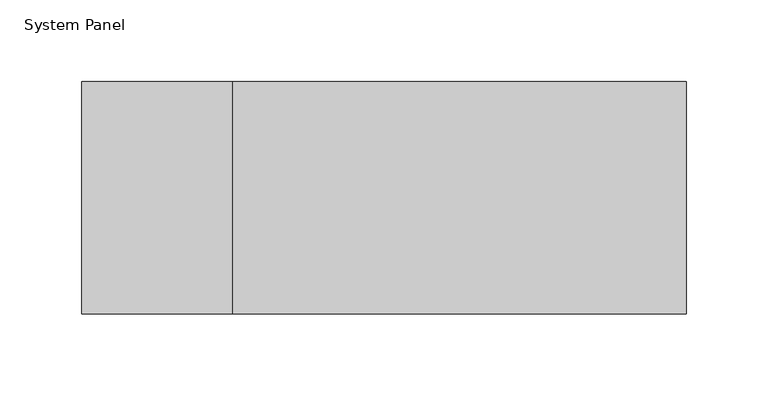
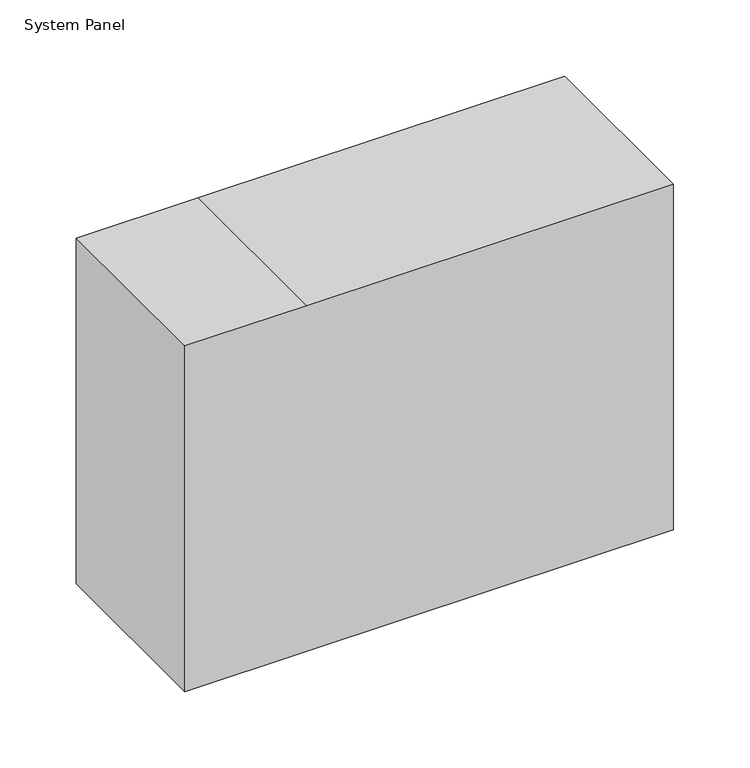
"""IFC4 building model written with IfcOpenShell, lengths in millimetres: plate geometry, System Panel : NLRS_21_CWP_hsb-vulling minerale wol 142 _gen_rsf."""

from ifc_helpers import new_model, si_unit, frame, origin, place, context, project, spatial, polyline, outline, extrude, source, transform, mapped, element, save


def system_panel_b83392b1(model_context):
    return source(origin(), model_context, "Body", "SweptSolid", [
        extrude(outline(polyline([(0.0, -184.5), (0.0, -92.5), (0.0, 184.5), (276.0, 184.5), (276.0, -92.5), (276.0, -184.5), (0.0, -184.5)])), frame((0.0, -71.0, 0.0), z_axis=(0.0, 1.0, 0.0), x_axis=(0.0, 0.0, 1.0)), (0.0, 0.0, 1.0), 142.0),
    ])


if __name__ == "__main__":
    model = new_model("IFC4")
    model_context = context("Model", 3, world=origin())
    ifc_project = project(units=[si_unit("LENGTHUNIT", "METRE", prefix="MILLI")], contexts=[model_context])
    site = spatial("IfcSite", under=ifc_project)
    building = spatial("IfcBuilding", under=site)
    placement = place(None, origin())
    system_panel_shape = system_panel_b83392b1(model_context)
    element("IfcPlate", 1, ObjectType="System Panel : NLRS_21_CWP_hsb-vulling minerale wol 142 _gen_rsf", at=placement, inside=building, context=model_context, shape_type="MappedRepresentation", body=[
        mapped(system_panel_shape, transform((0.0, 0.0, 0.0), x_axis=(1.0, 0.0, 0.0), y_axis=(0.0, 1.0, 0.0), z_axis=(0.0, 0.0, 1.0))),
    ])
    save(model, "model.ifc")

# Revit data of these elements
# Type "System Panel : NLRS_21_CWP_hsb-vulling minerale wol 142 _gen_rsf"
#   Export Type to IFC As = "IfcWall"
#   Type IfcGUID = "07M7mRoiH1CR8m_RSKIwpC"
#   Assembly Code = "21.23"
# Element 1 (IfcPlate, "System Panel : NLRS_21_CWP_hsb-vulling minerale wol 142 _gen_rsf")
#   Materials on its faces: "NLRS_m1_isolatie minerale wol_gen_rsf"
# Materials
#   "NLRS_m1_isolatie minerale wol_gen_rsf": class "M - Anorganische materialen", colour RGB 200 200 140, transparency 0, Keynote = "m1", Manufacturer = "Revit Standards Foundation", URL = "www.revitstandards.org", Description = "isolatie minerale wol", Cost = 0
